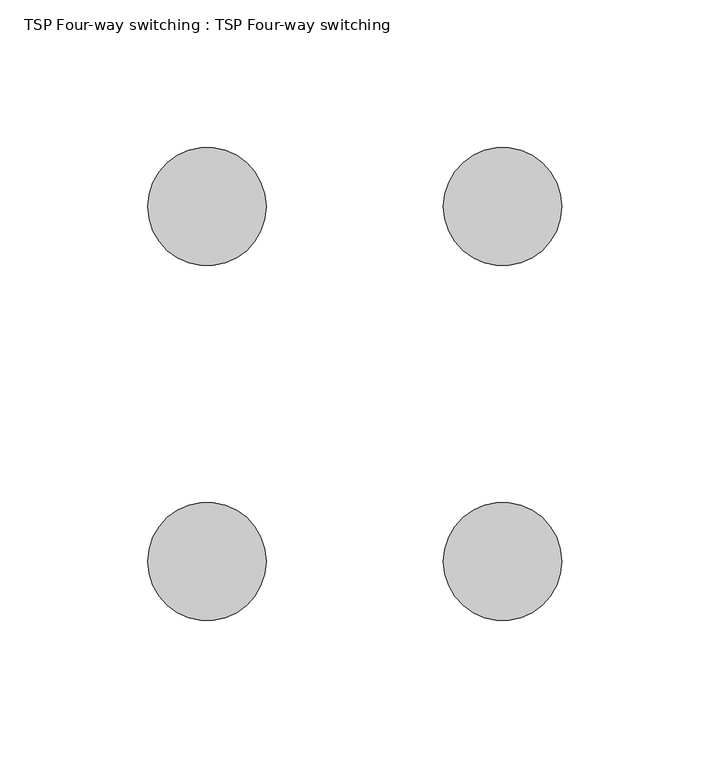
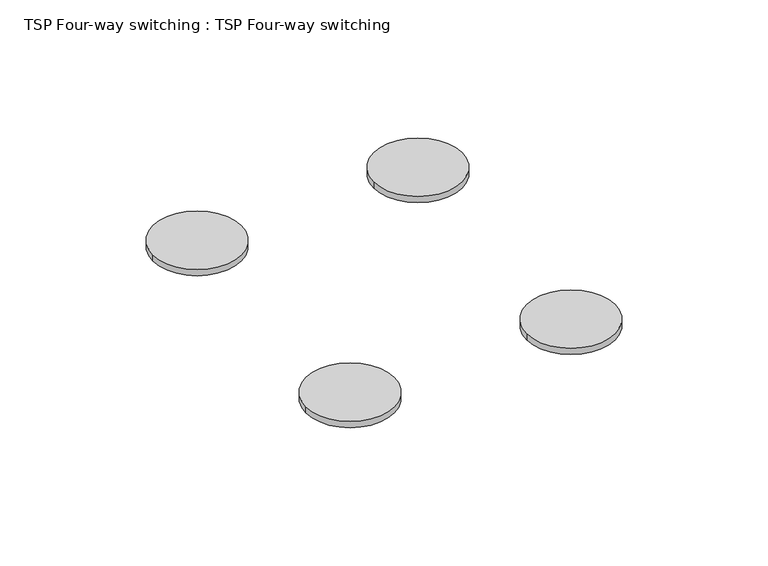
"""IFC4 building model written with IfcOpenShell, lengths in millimetres: proxy geometry, TSP Four-way switching : TSP Four-way switching."""

from ifc_helpers import new_model, si_unit, point, frame_2d, origin, origin_with_axes, place, context, project, spatial, circle_curve, trimmed, segment, composite_curve, outline, extrude, source, transform, mapped, element, save


def tsp_four_way_switching_tsp_four_way_switching_415c368a(model_context):
    return source(origin(), model_context, "Body", "SweptSolid", [
        extrude(outline(composite_curve([segment(trimmed(circle_curve(frame_2d((50.0, 60.0)), 20.0), [point((70.0, 60.0))], [point((30.0, 60.0))], False, "CARTESIAN"), True, "CONTINUOUS"), segment(trimmed(circle_curve(frame_2d((50.0, 60.0)), 20.0), [point((30.0, 60.0))], [point((70.0, 60.0))], False, "CARTESIAN"), True, "CONTINUOUS")], self_intersect=False)), origin_with_axes(), (0.0, 0.0, 1.0), 3.0),
        extrude(outline(composite_curve([segment(trimmed(circle_curve(frame_2d((-50.0, -60.0)), 20.0), [point((-70.0, -60.0))], [point((-30.0, -60.0))], False, "CARTESIAN"), True, "CONTINUOUS"), segment(trimmed(circle_curve(frame_2d((-50.0, -60.0)), 20.0), [point((-30.0, -60.0))], [point((-70.0, -60.0))], False, "CARTESIAN"), True, "CONTINUOUS")], self_intersect=False)), origin_with_axes(), (0.0, 0.0, 1.0), 3.0),
        extrude(outline(composite_curve([segment(trimmed(circle_curve(frame_2d((50.0, -60.0)), 20.0), [point((70.0, -60.0))], [point((30.0, -60.0))], False, "CARTESIAN"), True, "CONTINUOUS"), segment(trimmed(circle_curve(frame_2d((50.0, -60.0)), 20.0), [point((30.0, -60.0))], [point((70.0, -60.0))], False, "CARTESIAN"), True, "CONTINUOUS")], self_intersect=False)), origin_with_axes(), (0.0, 0.0, 1.0), 3.0),
        extrude(outline(composite_curve([segment(trimmed(circle_curve(frame_2d((-50.0, 60.0)), 20.0), [point((-70.0, 60.0))], [point((-30.0, 60.0))], False, "CARTESIAN"), True, "CONTINUOUS"), segment(trimmed(circle_curve(frame_2d((-50.0, 60.0)), 20.0), [point((-30.0, 60.0))], [point((-70.0, 60.0))], False, "CARTESIAN"), True, "CONTINUOUS")], self_intersect=False)), origin_with_axes(), (0.0, 0.0, 1.0), 3.0),
    ])


if __name__ == "__main__":
    model = new_model("IFC4")
    model_context = context("Model", 3, world=origin())
    ifc_project = project(units=[si_unit("LENGTHUNIT", "METRE", prefix="MILLI")], contexts=[model_context])
    site = spatial("IfcSite", under=ifc_project)
    building = spatial("IfcBuilding", under=site)
    placement = place(None, origin())
    tsp_four_way_switching_tsp_four_way_switching_shape = tsp_four_way_switching_tsp_four_way_switching_415c368a(model_context)
    element("IfcBuildingElementProxy", 1, Name="TSP Four-way switching : TSP Four-way switching", ObjectType="TSP Four-way switching : TSP Four-way switching", at=placement, inside=building, context=model_context, shape_type="MappedRepresentation", body=[
        mapped(tsp_four_way_switching_tsp_four_way_switching_shape, transform((0.0, 0.0, 0.0), x_axis=(1.0, 0.0, 0.0), y_axis=(0.0, 1.0, 0.0), z_axis=(0.0, 0.0, 1.0))),
    ])
    save(model, "model.ifc")

# Revit data of these elements
# Type "TSP Four-way switching : TSP Four-way switching"
#   Model = "TSP_ELEC4WS"
#   Default Elevation = 0
# Element 1 (IfcBuildingElementProxy, "TSP Four-way switching : TSP Four-way switching")
#   Materials on its faces: "Plastic, Opaque Black"
# Materials
#   "Plastic, Opaque Black": class "Plastic", colour RGB 0 0 0, transparency 0.7, Description = "Plastic, generic, opaque black", Cost = 0
